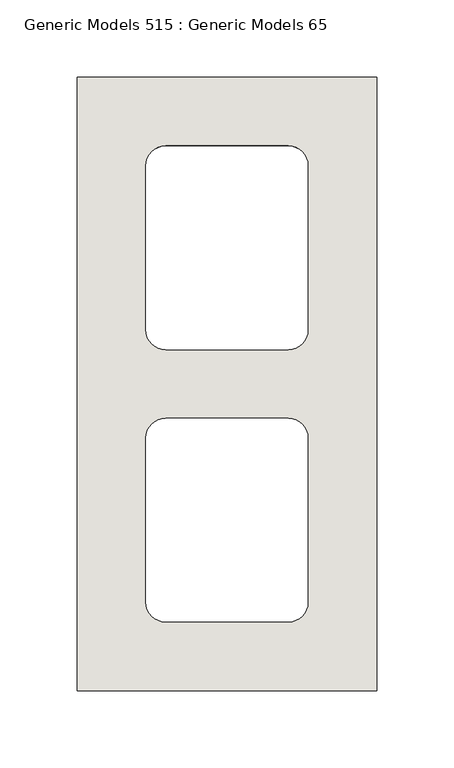
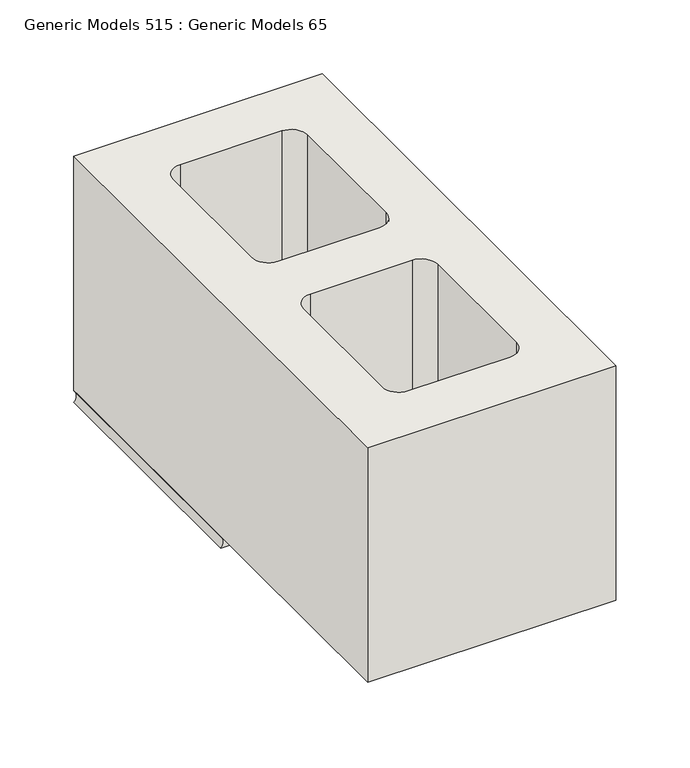
"""IFC4 building model written with IfcOpenShell, lengths in millimetres: wall geometry, Generic Models 515 : Generic Models 65."""

from ifc_helpers import new_model, si_unit, point, frame, frame_2d, origin, place, context, project, spatial, polyline, circle_curve, trimmed, segment, composite_curve, outline, extrude, source, transform, mapped, element, save
from ifc_brep_helpers import plane_surface, revolved_surface, advanced_brep


def generic_models_515_generic_models_65_243d8d1a(model_context):
    return source(origin(), model_context, "Body", "SolidModel", [
        advanced_brep(
        [(428979.0125, 503.2375, 9.525), (428785.3375, 503.2375, 9.525), (428785.3375, 503.2375, 0.0), (428979.0125, 503.2375, 0.0), (428979.0125, 701.675, 9.525), (428979.0125, 701.675, 0.0), (428785.3375, 701.675, 0.0), (428785.3375, 701.675, 9.525), (428934.5625, 538.1625, 9.525), (428921.8625, 525.4625, 9.525), (428842.4875, 525.4625, 9.525), (428829.7875, 538.1625, 9.525), (428829.7875, 644.525, 9.525), (428842.4875, 657.225, 9.525), (428921.8625, 657.225, 9.525), (428934.5625, 644.525, 9.525), (428921.8625, 525.4625, 0.0), (428934.5625, 538.1625, 0.0), (428842.4875, 525.4625, 0.0), (428829.7875, 538.1625, 0.0), (428829.7875, 644.525, 0.0), (428842.4875, 657.225, 0.0), (428921.8625, 657.225, 0.0), (428934.5625, 644.525, 0.0)],
        [
            (0, 1),
            (1, 2, circle_curve(frame((428780.4545028, 503.2375, 4.7625), z_axis=(0.0, 1.0, 0.0), x_axis=(1.0, 0.0, 0.0)), 6.8209287)),
            (2, 3),
            (3, 0, circle_curve(frame((428983.8954972, 503.2375, 4.7625), z_axis=(0.0, 1.0, 0.0), x_axis=(-1.0, 0.0, 0.0)), 6.8209287)),
            (4, 5, circle_curve(frame((428983.8954972, 701.675, 4.7625), z_axis=(0.0, -1.0, 0.0), x_axis=(-1.0, 0.0, 0.0)), 6.8209287)),
            (5, 6),
            (6, 7, circle_curve(frame((428780.4545028, 701.675, 4.7625), z_axis=(0.0, -1.0, 0.0), x_axis=(1.0, 0.0, 0.0)), 6.8209287)),
            (7, 4),
            (0, 4),
            (7, 1),
            (8, 9, circle_curve(frame((428921.8625, 538.1625, 9.525), z_axis=(0.0, 0.0, -1.0), x_axis=(-1.0, 0.0, 0.0)), 12.7)),
            (9, 10),
            (10, 11, circle_curve(frame((428842.4875, 538.1625, 9.525), z_axis=(0.0, 0.0, -1.0), x_axis=(-1.0, 0.0, 0.0)), 12.7)),
            (11, 12),
            (12, 13, circle_curve(frame((428842.4875, 644.525, 9.525), z_axis=(0.0, 0.0, -1.0), x_axis=(-1.0, 0.0, 0.0)), 12.7)),
            (13, 14),
            (14, 15, circle_curve(frame((428921.8625, 644.525, 9.525), z_axis=(0.0, 0.0, -1.0), x_axis=(-1.0, 0.0, 0.0)), 12.7)),
            (15, 8),
            (16, 9),
            (8, 17),
            (17, 16, circle_curve(frame((428921.8625, 538.1625, 0.0), z_axis=(0.0, 0.0, -1.0), x_axis=(-1.0, 0.0, 0.0)), 12.7)),
            (16, 18),
            (18, 10),
            (18, 19, circle_curve(frame((428842.4875, 538.1625, 0.0), z_axis=(0.0, 0.0, -1.0), x_axis=(-1.0, 0.0, 0.0)), 12.7)),
            (19, 11),
            (19, 20),
            (20, 12),
            (20, 21, circle_curve(frame((428842.4875, 644.525, 0.0), z_axis=(0.0, 0.0, -1.0), x_axis=(-1.0, 0.0, 0.0)), 12.7)),
            (21, 13),
            (21, 22),
            (22, 14),
            (22, 23, circle_curve(frame((428921.8625, 644.525, 0.0), z_axis=(0.0, 0.0, -1.0), x_axis=(-1.0, 0.0, 0.0)), 12.7)),
            (23, 15),
            (23, 17),
            (6, 2),
            (5, 3),
        ],
        [
            plane_surface(frame((428882.175, 503.2375, 9.921875), z_axis=(0.0, -1.0, 0.0), x_axis=(0.0, 0.0, 1.0))),
            plane_surface(frame((428882.175, 701.675, 9.921875), z_axis=(0.0, 1.0, 0.0), x_axis=(0.0, 0.0, 1.0))),
            plane_surface(frame((428979.0125, 503.2375, 9.525), z_axis=(0.0, 0.0, 1.0), x_axis=(0.0, 1.0, 0.0))),
            revolved_surface(polyline([(428909.1625, 538.1625, 9.525000000000006), (428909.1625, 538.1625, 0.0)]), (428921.8625, 538.1625, 193.675), (0.0, 0.0, 1.0)),
            plane_surface(frame((428842.4875, 525.4625, 193.675), z_axis=(0.0, 1.0, 0.0), x_axis=(0.0, 0.0, -1.0))),
            revolved_surface(polyline([(428829.7875, 538.1625, 9.525000000000006), (428829.7875, 538.1625, 0.0)]), (428842.4875, 538.1625, 193.675), (0.0, 0.0, 1.0)),
            plane_surface(frame((428829.7875, 644.525, 193.675), z_axis=(1.0, 0.0, 0.0), x_axis=(0.0, 0.0, -1.0))),
            revolved_surface(polyline([(428829.7875, 644.525, 9.525000000000006), (428829.7875, 644.525, 0.0)]), (428842.4875, 644.525, 193.675), (0.0, 0.0, 1.0)),
            plane_surface(frame((428921.8625, 657.225, 193.675), z_axis=(0.0, -1.0, 0.0), x_axis=(0.0, 0.0, -1.0))),
            revolved_surface(polyline([(428909.1625, 644.525, 9.525000000000006), (428909.1625, 644.525, 0.0)]), (428921.8625, 644.525, 193.675), (0.0, 0.0, 1.0)),
            plane_surface(frame((428934.5625, 538.1625, 193.675), z_axis=(-1.0, 0.0, 0.0), x_axis=(0.0, 0.0, -1.0))),
            revolved_surface(polyline([(428787.2754315, 701.675, 4.7625), (428787.2754315, 503.2375, 4.7625)]), (428780.4545028, 503.2375, 4.7625), (0.0, 1.0, 0.0)),
            plane_surface(frame((428785.3375, 503.2375, 0.0), z_axis=(0.0, 0.0, -1.0), x_axis=(0.0, 1.0, 0.0))),
            revolved_surface(polyline([(428977.07456850004, 701.675, 4.7625), (428977.07456850004, 503.2375, 4.7625)]), (428983.8954972, 503.2375, 4.7625), (0.0, 1.0, 0.0)),
        ],
        [
            (0, [[1, 2, 3, 4]]),
            (1, [[5, 6, 7, 8]]),
            (2, [[-1, 9, -8, 10], [11, 12, 13, 14, 15, 16, 17, 18]]),
            (3, [[19, -11, 20, 21]]),
            (4, [[-19, 22, 23, -12]]),
            (5, [[-23, 24, 25, -13]]),
            (6, [[-25, 26, 27, -14]]),
            (7, [[-27, 28, 29, -15]]),
            (8, [[-29, 30, 31, -16]]),
            (9, [[-31, 32, 33, -17]]),
            (10, [[-33, 34, -20, -18]]),
            (11, [[-2, -10, -7, 35]]),
            (12, [[-3, -35, -6, 36], [-21, -34, -32, -30, -28, -26, -24, -22]]),
            (13, [[-4, -36, -5, -9]]),
        ],
    ),
        extrude(outline(polyline([(428979.0125, 304.8), (428785.3375, 304.8), (428785.3375, 701.675), (428979.0125, 701.675), (428979.0125, 304.8)]), holes=[composite_curve([segment(polyline([(428934.5625, 538.1625), (428934.5625, 644.525)]), True, "CONTINUOUS"), segment(trimmed(circle_curve(frame_2d((428921.8625, 644.525)), 12.7), [point((428934.5625, 644.525))], [point((428921.8625, 657.225))], True, "CARTESIAN"), True, "CONTINUOUS"), segment(polyline([(428921.8625, 657.225), (428842.4875, 657.225)]), True, "CONTINUOUS"), segment(trimmed(circle_curve(frame_2d((428842.4875, 644.525)), 12.7), [point((428842.4875, 657.225))], [point((428829.7875, 644.525))], True, "CARTESIAN"), True, "CONTINUOUS"), segment(polyline([(428829.7875, 644.525), (428829.7875, 538.1625)]), True, "CONTINUOUS"), segment(trimmed(circle_curve(frame_2d((428842.4875, 538.1625)), 12.7), [point((428829.7875, 538.1625))], [point((428842.4875, 525.4625))], True, "CARTESIAN"), True, "CONTINUOUS"), segment(polyline([(428842.4875, 525.4625), (428921.8625, 525.4625)]), True, "CONTINUOUS"), segment(trimmed(circle_curve(frame_2d((428921.8625, 538.1625)), 12.7), [point((428921.8625, 525.4625))], [point((428934.5625, 538.1625))], True, "CARTESIAN"), True, "CONTINUOUS")], self_intersect=False), composite_curve([segment(polyline([(428829.7875, 468.3125), (428829.7875, 361.95)]), True, "CONTINUOUS"), segment(trimmed(circle_curve(frame_2d((428842.4875, 361.95)), 12.7), [point((428829.7875, 361.95))], [point((428842.4875, 349.25))], True, "CARTESIAN"), True, "CONTINUOUS"), segment(polyline([(428842.4875, 349.25), (428921.8625, 349.25)]), True, "CONTINUOUS"), segment(trimmed(circle_curve(frame_2d((428921.8625, 361.95)), 12.7), [point((428921.8625, 349.25))], [point((428934.5625, 361.95))], True, "CARTESIAN"), True, "CONTINUOUS"), segment(polyline([(428934.5625, 361.95), (428934.5625, 468.3125)]), True, "CONTINUOUS"), segment(trimmed(circle_curve(frame_2d((428921.8625, 468.3125)), 12.7), [point((428934.5625, 468.3125))], [point((428921.8625, 481.0125))], True, "CARTESIAN"), True, "CONTINUOUS"), segment(polyline([(428921.8625, 481.0125), (428842.4875, 481.0125)]), True, "CONTINUOUS"), segment(trimmed(circle_curve(frame_2d((428842.4875, 468.3125)), 12.7), [point((428842.4875, 481.0125))], [point((428829.7875, 468.3125))], True, "CARTESIAN"), True, "CONTINUOUS")], self_intersect=False)]), frame((0.0, 0.0, 9.525), z_axis=(0.0, 0.0, 1.0), x_axis=(1.0, 0.0, 0.0)), (0.0, 0.0, 1.0), 193.675),
    ])


if __name__ == "__main__":
    model = new_model("IFC4")
    model_context = context("Model", 3, world=origin())
    ifc_project = project(units=[si_unit("LENGTHUNIT", "METRE", prefix="MILLI")], contexts=[model_context])
    site = spatial("IfcSite", under=ifc_project)
    building = spatial("IfcBuilding", under=site)
    placement = place(None, origin())
    generic_models_515_generic_models_65_shape = generic_models_515_generic_models_65_243d8d1a(model_context)
    element("IfcWall", 1, ObjectType="Generic Models 515 : Generic Models 65", at=placement, inside=building, context=model_context, shape_type="MappedRepresentation", body=[
        mapped(generic_models_515_generic_models_65_shape, transform((0.0, 0.0, 0.0), x_axis=(1.0, 0.0, 0.0), y_axis=(0.0, 1.0, 0.0), z_axis=(0.0, 0.0, 1.0))),
    ])
    save(model, "model.ifc")

# Revit data of these elements
# Element 1 (IfcWall, "Generic Models 515 : Generic Models 65")
#   Materials on its faces: "CMU (SEE 'WALL TAG' FOR SIZE)", "MORTAR JOINT"
# Materials
#   "CMU (SEE 'WALL TAG' FOR SIZE)": class "Masonry", colour RGB 203 203 199, transparency 0, Description = "Concrete masonry units", Cost = 0
#   "MORTAR JOINT": class "Generic", colour RGB 120 120 120, transparency 0, Cost = 0
